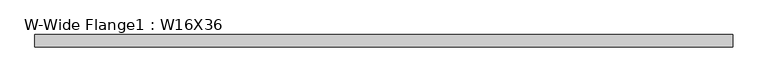
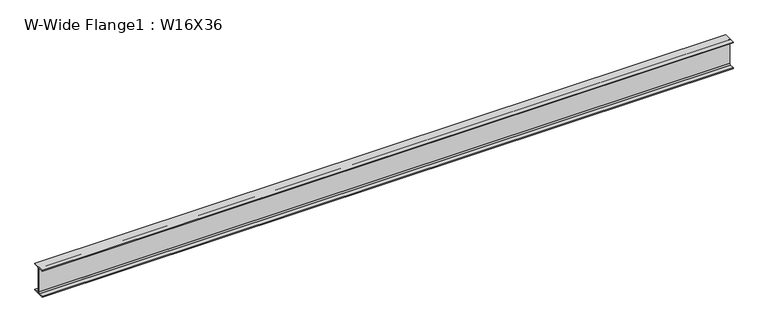
"""IFC4 building model written with IfcOpenShell, lengths in millimetres: beam geometry, W-Wide Flange1 : W16X36."""

from ifc_helpers import new_model, si_unit, point, frame, frame_2d, origin, place, context, project, spatial, polyline, circle_curve, trimmed, segment, composite_curve, outline, extrude, source, transform, mapped, element, save


def w_wide_flange1_w16x36_0cb94c8a(model_context):
    return source(origin(), model_context, "Body", "SweptSolid", [
        extrude(outline(composite_curve([segment(polyline([(88.773, -191.008), (88.773, -201.93), (-88.773, -201.93), (-88.773, -191.008), (-21.3995, -191.008)]), True, "CONTINUOUS"), segment(trimmed(circle_curve(frame_2d((-21.3995, -173.355)), 17.653), [point((-21.3995, -191.008))], [point((-3.7465, -173.355))], True, "CARTESIAN"), True, "CONTINUOUS"), segment(polyline([(-3.7465, -173.355), (-3.7465, 173.355)]), True, "CONTINUOUS"), segment(trimmed(circle_curve(frame_2d((-21.3995, 173.355)), 17.653), [point((-3.7465, 173.355))], [point((-21.3995, 191.008))], True, "CARTESIAN"), True, "CONTINUOUS"), segment(polyline([(-21.3995, 191.008), (-88.773, 191.008), (-88.773, 201.93), (88.773, 201.93), (88.773, 191.008), (21.3995, 191.008)]), True, "CONTINUOUS"), segment(trimmed(circle_curve(frame_2d((21.3995, 173.355)), 17.653), [point((21.3995, 191.008))], [point((3.7465, 173.355))], True, "CARTESIAN"), True, "CONTINUOUS"), segment(polyline([(3.7465, 173.355), (3.7465, -173.355)]), True, "CONTINUOUS"), segment(trimmed(circle_curve(frame_2d((21.3995, -173.355)), 17.653), [point((3.7465, -173.355))], [point((21.3995, -191.008))], True, "CARTESIAN"), True, "CONTINUOUS"), segment(polyline([(21.3995, -191.008), (88.773, -191.008)]), True, "CONTINUOUS")], self_intersect=False)), frame((-4997.6202708, 0.0, 0.0), z_axis=(1.0, 0.0, 0.0), x_axis=(0.0, 1.0, 0.0)), (0.0, 0.0, 1.0), 9898.6362057),
    ])


if __name__ == "__main__":
    model = new_model("IFC4")
    model_context = context("Model", 3, world=origin())
    ifc_project = project(units=[si_unit("LENGTHUNIT", "METRE", prefix="MILLI")], contexts=[model_context])
    site = spatial("IfcSite", under=ifc_project)
    building = spatial("IfcBuilding", under=site)
    placement = place(None, origin())
    w_wide_flange1_w16x36_shape = w_wide_flange1_w16x36_0cb94c8a(model_context)
    element("IfcBeam", 1, ObjectType="W-Wide Flange1 : W16X36", at=placement, inside=building, context=model_context, shape_type="MappedRepresentation", body=[
        mapped(w_wide_flange1_w16x36_shape, transform((0.0, 0.0, 0.0), x_axis=(1.0, 0.0, 0.0), y_axis=(0.0, 1.0, 0.0), z_axis=(0.0, 0.0, 1.0))),
    ])
    save(model, "model.ifc")

# Revit data of these elements
# Type "W-Wide Flange1 : W16X36"
#   Assembly Code = "B10"
#   W = 36
#   Start Extension Calculation [instance default] = 10' - 0"
#   Start Extension [instance default] = -0' - 0 1/2"
#   End Extension Calculation [instance default] = 10' - 0"
#   End Extension [instance default] = -0' - 0 1/2"
#   Length [instance default] = 5' - 0"
#   bf = 0' - 6.99"
#   d = 1' - 3.9"
#   k = 0' - 1 1/8"
#   k2 = 0' - 0.695"
#   tf = 0' - 0.43"
#   tw = 0' - 0.295"
#   A = 0.0736111 SF
#   Structural Material [instance default] = Metal - Steel - ASTM A992
# Element 1 (IfcBeam, "W-Wide Flange1 : W16X36")
#   Materials on its faces: "Metal - Steel - ASTM A992"
# Materials
#   "Metal - Steel - ASTM A992": class "Metal", colour RGB 199 199 199, transparency 0
